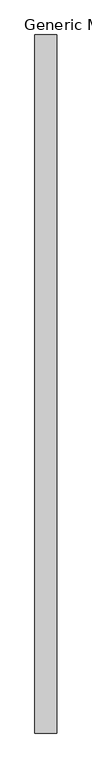
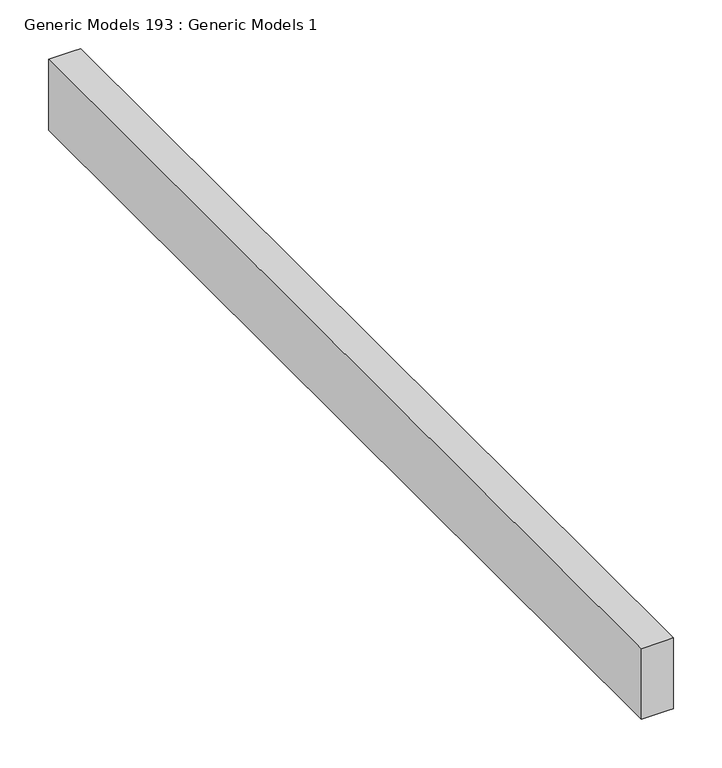
"""IFC4 building model written with IfcOpenShell, lengths in millimetres: proxy geometry, Generic Models 193 : Generic Models 1."""

from ifc_helpers import new_model, si_unit, origin, place, context, project, spatial, faceted_brep, source, transform, mapped, element, save


def generic_models_193_generic_models_1_5d5b5675(model_context):
    return source(origin(), model_context, "Body", "Brep", [
        faceted_brep([(47345.6, 0.0, 380.0195631), (47337.6625, 0.0, 380.0195631), (47307.5, 0.0, 380.0195631), (47307.5, 0.0, 291.1195631), (47337.6625, 0.0, 291.1195631), (47345.6, 0.0, 291.1195631), (47345.6, 1219.2, 380.0195631), (47345.6, 1219.2, 291.1195631), (47337.6625, 1219.2, 291.1195631), (47307.5, 1219.2, 291.1195631), (47307.5, 1219.2, 380.0195631), (47337.6625, 1219.2, 380.0195631)], [[[0, 1, 2, 3, 4, 5]], [[6, 7, 8, 9, 10, 11]], [[5, 4, 3, 9, 8, 7]], [[3, 2, 10, 9]], [[2, 1, 0, 6, 11, 10]], [[0, 5, 7, 6]]]),
    ])


if __name__ == "__main__":
    model = new_model("IFC4")
    model_context = context("Model", 3, world=origin())
    ifc_project = project(units=[si_unit("LENGTHUNIT", "METRE", prefix="MILLI")], contexts=[model_context])
    site = spatial("IfcSite", under=ifc_project)
    building = spatial("IfcBuilding", under=site)
    placement = place(None, origin())
    generic_models_193_generic_models_1_shape = generic_models_193_generic_models_1_5d5b5675(model_context)
    element("IfcBuildingElementProxy", 1, Name="Generic Models 193 : Generic Models 1", ObjectType="Generic Models 193 : Generic Models 1", at=placement, inside=building, context=model_context, shape_type="MappedRepresentation", body=[
        mapped(generic_models_193_generic_models_1_shape, transform((0.0, 0.0, 0.0), x_axis=(1.0, 0.0, 0.0), y_axis=(0.0, 1.0, 0.0), z_axis=(0.0, 0.0, 1.0))),
    ])
    save(model, "model.ifc")

# Revit data of these elements
# Element 1 (IfcBuildingElementProxy, "Generic Models 193 : Generic Models 1")
#   Materials on its faces: "2X BLOCKING - LOCATED AT GRAB BARS, WALL HUNG CABINETS, ETC.)"
# Materials
#   "2X BLOCKING - LOCATED AT GRAB BARS, WALL HUNG CABINETS, ETC.)": class "Wood", colour RGB 234 198 147, transparency 0, Description = "Pinus Echinata", Cost = 0
